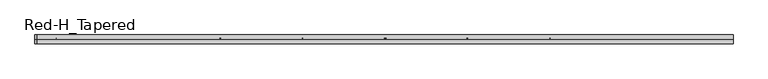
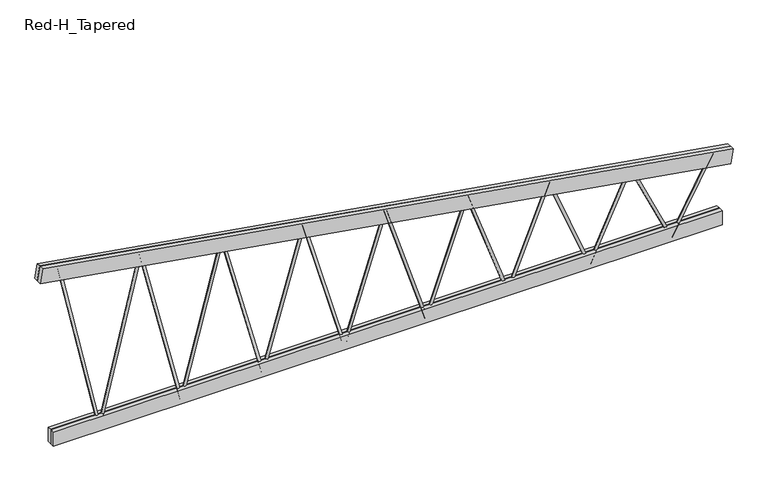
"""IFC4 building model written with IfcOpenShell, lengths in millimetres: beam geometry, Construction_Frames_RedBuilt_Openweb_Red-H_Tapered : Red-H_Tapered."""

from ifc_helpers import new_model, si_unit, point, frame, origin, origin_2d, place, context, project, spatial, polyline, circle_curve, trimmed, segment, composite_curve, outline, extrude, source, transform, mapped, element, save


def red_h_tapered_2805eec2(model_context):
    return source(origin(), model_context, "Body", "SweptSolid", [
        extrude(outline(composite_curve([segment(trimmed(circle_curve(origin_2d(), 12.7), [point((0.0, -12.7))], [point((0.0, 12.7))], False, "CARTESIAN"), True, "CONTINUOUS"), segment(trimmed(circle_curve(origin_2d(), 12.7), [point((0.0, 12.7))], [point((0.0, -12.7))], False, "CARTESIAN"), True, "CONTINUOUS")], self_intersect=False)), frame((-378.61875, 0.0, -417.8101562), z_axis=(-0.277995532529411, 0.0, 0.9605823670532836), x_axis=(0.0, 1.0, 0.0)), (0.0, 0.0, 1.0), 1361.9598364),
        extrude(outline(composite_curve([segment(trimmed(circle_curve(origin_2d(), 12.7), [point((0.0, 12.7))], [point((0.0, -12.7))], False, "CARTESIAN"), True, "CONTINUOUS"), segment(trimmed(circle_curve(origin_2d(), 12.7), [point((0.0, -12.7))], [point((0.0, 12.7))], False, "CARTESIAN"), True, "CONTINUOUS")], self_intersect=False)), frame((-1135.85625, 0.0, -417.8101562), z_axis=(0.27799553252941006, 0.0, 0.9605823670532838), x_axis=(0.0, 1.0, 0.0)), (0.0, 0.0, 1.0), 1361.9598364),
        extrude(outline(composite_curve([segment(trimmed(circle_curve(origin_2d(), 12.7), [point((0.0, -12.7))], [point((0.0, 12.7000001))], False, "CARTESIAN"), True, "CONTINUOUS"), segment(trimmed(circle_curve(origin_2d(), 12.7), [point((0.0, 12.7000001))], [point((0.0, -12.7))], False, "CARTESIAN"), True, "CONTINUOUS")], self_intersect=False)), frame((-1135.85625, 0.0, -417.8101562), z_axis=(-0.2554865755688276, 0.0, 0.966812603198838), x_axis=(0.0, 1.0, 0.0)), (0.0, 0.0, 1.0), 1481.9516413),
        extrude(outline(composite_curve([segment(trimmed(circle_curve(origin_2d(), 12.7), [point((0.0, 12.7))], [point((0.0, -12.7000001))], False, "CARTESIAN"), True, "CONTINUOUS"), segment(trimmed(circle_curve(origin_2d(), 12.7), [point((0.0, -12.7000001))], [point((0.0, 12.7))], False, "CARTESIAN"), True, "CONTINUOUS")], self_intersect=False)), frame((-1893.09375, 0.0, -417.8101562), z_axis=(0.25548657556883586, 0.0, 0.9668126031988359), x_axis=(0.0, 1.0, 0.0)), (0.0, 0.0, 1.0), 1481.9516413),
        extrude(outline(composite_curve([segment(trimmed(circle_curve(origin_2d(), 12.7), [point((0.0, -12.7))], [point((0.0, 12.7))], False, "CARTESIAN"), True, "CONTINUOUS"), segment(trimmed(circle_curve(origin_2d(), 12.7), [point((0.0, 12.7))], [point((0.0, -12.7))], False, "CARTESIAN"), True, "CONTINUOUS")], self_intersect=False)), frame((-1893.09375, 0.0, -417.8101562), z_axis=(-0.23624830304325084, 0.0, 0.9716927185634275), x_axis=(0.0, 1.0, 0.0)), (0.0, 0.0, 1.0), 1602.6305591),
        extrude(outline(composite_curve([segment(trimmed(circle_curve(origin_2d(), 12.7), [point((0.0, 12.7))], [point((0.0, -12.7))], False, "CARTESIAN"), True, "CONTINUOUS"), segment(trimmed(circle_curve(origin_2d(), 12.7), [point((0.0, -12.7))], [point((0.0, 12.7))], False, "CARTESIAN"), True, "CONTINUOUS")], self_intersect=False)), frame((-2650.33125, 0.0, -417.8101562), z_axis=(0.23624830304324398, 0.0, 0.9716927185634292), x_axis=(0.0, 1.0, 0.0)), (0.0, 0.0, 1.0), 1602.6305591),
        extrude(outline(composite_curve([segment(trimmed(circle_curve(origin_2d(), 12.7), [point((0.0, -12.7))], [point((0.0, 12.7))], False, "CARTESIAN"), True, "CONTINUOUS"), segment(trimmed(circle_curve(origin_2d(), 12.7), [point((0.0, 12.7))], [point((0.0, -12.7))], False, "CARTESIAN"), True, "CONTINUOUS")], self_intersect=False)), frame((-2650.33125, 0.0, -417.8101562), z_axis=(-0.21963526223165897, 0.0, 0.9755820578426145), x_axis=(0.0, 1.0, 0.0)), (0.0, 0.0, 1.0), 1723.8522911),
        extrude(outline(composite_curve([segment(trimmed(circle_curve(origin_2d(), 12.7), [point((0.0, -12.7))], [point((0.0, 12.7))], False, "CARTESIAN"), True, "CONTINUOUS"), segment(trimmed(circle_curve(origin_2d(), 12.7), [point((0.0, 12.7))], [point((0.0, -12.7))], False, "CARTESIAN"), True, "CONTINUOUS")], self_intersect=False)), frame((2650.33125, 0.0, -417.8101562), z_axis=(0.48331839774277513, 0.0, 0.8754446449681195), x_axis=(0.0, 1.0, 0.0)), (0.0, 0.0, 1.0), 783.3733451),
        extrude(outline(composite_curve([segment(trimmed(circle_curve(origin_2d(), 12.7), [point((0.0, 12.7))], [point((0.0, -12.7))], False, "CARTESIAN"), True, "CONTINUOUS"), segment(trimmed(circle_curve(origin_2d(), 12.7), [point((0.0, -12.7))], [point((0.0, 12.7))], False, "CARTESIAN"), True, "CONTINUOUS")], self_intersect=False)), frame((2650.33125, 0.0, -417.8101562), z_axis=(-0.4233271479189003, 0.0, 0.9059768903426011), x_axis=(0.0, 1.0, 0.0)), (0.0, 0.0, 1.0), 894.3880681),
        extrude(outline(composite_curve([segment(trimmed(circle_curve(origin_2d(), 12.7), [point((0.0, -12.7))], [point((0.0, 12.7))], False, "CARTESIAN"), True, "CONTINUOUS"), segment(trimmed(circle_curve(origin_2d(), 12.7), [point((0.0, 12.7))], [point((0.0, -12.7))], False, "CARTESIAN"), True, "CONTINUOUS")], self_intersect=False)), frame((1893.09375, 0.0, -417.8101562), z_axis=(0.42332714791889964, 0.0, 0.9059768903426014), x_axis=(0.0, 1.0, 0.0)), (0.0, 0.0, 1.0), 894.3880681),
        extrude(outline(composite_curve([segment(trimmed(circle_curve(origin_2d(), 12.7), [point((0.0, 12.7))], [point((0.0, -12.7))], False, "CARTESIAN"), True, "CONTINUOUS"), segment(trimmed(circle_curve(origin_2d(), 12.7), [point((0.0, -12.7))], [point((0.0, 12.7))], False, "CARTESIAN"), True, "CONTINUOUS")], self_intersect=False)), frame((1893.09375, 0.0, -417.8101562), z_axis=(-0.3754069541599523, 0.0, 0.9268600858642838), x_axis=(0.0, 1.0, 0.0)), (0.0, 0.0, 1.0), 1008.5555044),
        extrude(outline(composite_curve([segment(trimmed(circle_curve(origin_2d(), 12.7), [point((0.0, -12.7))], [point((0.0, 12.7))], False, "CARTESIAN"), True, "CONTINUOUS"), segment(trimmed(circle_curve(origin_2d(), 12.7), [point((0.0, 12.7))], [point((0.0, -12.7))], False, "CARTESIAN"), True, "CONTINUOUS")], self_intersect=False)), frame((1135.85625, 0.0, -417.8101562), z_axis=(0.37540695415995146, 0.0, 0.9268600858642841), x_axis=(0.0, 1.0, 0.0)), (0.0, 0.0, 1.0), 1008.5555044),
        extrude(outline(composite_curve([segment(trimmed(circle_curve(origin_2d(), 12.7), [point((0.0, 12.7))], [point((0.0, -12.7))], False, "CARTESIAN"), True, "CONTINUOUS"), segment(trimmed(circle_curve(origin_2d(), 12.7), [point((0.0, -12.7))], [point((0.0, 12.7))], False, "CARTESIAN"), True, "CONTINUOUS")], self_intersect=False)), frame((1135.85625, 0.0, -417.8101562), z_axis=(-0.3365750833372033, 0.0, 0.9416566323647674), x_axis=(0.0, 1.0, 0.0)), (0.0, 0.0, 1.0), 1124.9161591),
        extrude(outline(composite_curve([segment(trimmed(circle_curve(origin_2d(), 12.7), [point((0.0, -12.7))], [point((0.0, 12.7))], False, "CARTESIAN"), True, "CONTINUOUS"), segment(trimmed(circle_curve(origin_2d(), 12.7), [point((0.0, 12.7))], [point((0.0, -12.7))], False, "CARTESIAN"), True, "CONTINUOUS")], self_intersect=False)), frame((378.61875, 0.0, -417.8101562), z_axis=(0.33657508333720376, 0.0, 0.9416566323647673), x_axis=(0.0, 1.0, 0.0)), (0.0, 0.0, 1.0), 1124.9161591),
        extrude(outline(composite_curve([segment(trimmed(circle_curve(origin_2d(), 12.7), [point((0.0, 12.7))], [point((0.0, -12.6999999))], False, "CARTESIAN"), True, "CONTINUOUS"), segment(trimmed(circle_curve(origin_2d(), 12.7), [point((0.0, -12.6999999))], [point((0.0, 12.7))], False, "CARTESIAN"), True, "CONTINUOUS")], self_intersect=False)), frame((378.61875, 0.0, -417.8101562), z_axis=(-0.3046365038173337, 0.0, 0.952468687433845), x_axis=(0.0, 1.0, 0.0)), (0.0, 0.0, 1.0), 1242.8541729),
        extrude(outline(composite_curve([segment(trimmed(circle_curve(origin_2d(), 12.7), [point((0.0, 12.6999999))], [point((0.0, -12.7))], False, "CARTESIAN"), True, "CONTINUOUS"), segment(trimmed(circle_curve(origin_2d(), 12.7), [point((0.0, -12.7))], [point((0.0, 12.6999999))], False, "CARTESIAN"), True, "CONTINUOUS")], self_intersect=False)), frame((-378.61875, 0.0, -417.8101562), z_axis=(0.30463650381731205, 0.0, 0.952468687433852), x_axis=(0.0, 1.0, 0.0)), (0.0, 0.0, 1.0), 1242.8541729),
        extrude(outline(polyline([(-3100.3875, 41.275), (3100.3875, 41.275), (3100.3875, 3.175), (-3100.3875, 3.175), (-3100.3875, 41.275)])), frame((0.0, 0.0, -436.8601562), z_axis=(0.0, 0.0, 1.0), x_axis=(1.0, 0.0, 0.0)), (0.0, 0.0, 1.0), 139.7),
        extrude(outline(polyline([(-3100.3875, -3.175), (3100.3875, -3.175), (3100.3875, -41.275), (-3100.3875, -41.275), (-3100.3875, -3.175)])), frame((0.0, 0.0, -436.8601562), z_axis=(0.0, 0.0, 1.0), x_axis=(1.0, 0.0, 0.0)), (0.0, 0.0, 1.0), 139.7),
        extrude(outline(polyline([(0.0, 38.1), (6492.222889, 38.1), (6492.222889, 0.0), (0.0, 0.0), (0.0, 38.1)])), frame((-3224.9429596, 3.175, 1203.3387666), z_axis=(0.16431968190823418, 0.0, 0.9864071381217681), x_axis=(0.9864071381217681, 0.0, -0.16431968190823418)), (0.0, 0.0, 1.0), 139.7),
        extrude(outline(polyline([(0.0, 38.1), (6492.222889, 38.1), (6492.222889, 0.0), (0.0, 0.0), (0.0, 38.1)])), frame((-3224.9429596, -41.275, 1203.3387666), z_axis=(0.16431968190823418, 0.0, 0.9864071381217681), x_axis=(0.9864071381217681, 0.0, -0.16431968190823418)), (0.0, 0.0, 1.0), 139.7),
    ])


if __name__ == "__main__":
    model = new_model("IFC4")
    model_context = context("Model", 3, world=origin())
    ifc_project = project(units=[si_unit("LENGTHUNIT", "METRE", prefix="MILLI")], contexts=[model_context])
    site = spatial("IfcSite", under=ifc_project)
    building = spatial("IfcBuilding", under=site)
    placement = place(None, origin())
    red_h_tapered_shape = red_h_tapered_2805eec2(model_context)
    element("IfcBeam", 1, ObjectType="Construction_Frames_RedBuilt_Openweb_Red-H_Tapered : Red-H_Tapered", at=placement, inside=building, context=model_context, shape_type="MappedRepresentation", body=[
        mapped(red_h_tapered_shape, transform((0.0, 0.0, 0.0), x_axis=(1.0, 0.0, 0.0), y_axis=(0.0, 1.0, 0.0), z_axis=(0.0, 0.0, 1.0))),
    ])
    save(model, "model.ifc")

# Revit data of these elements
# Type "Construction_Frames_RedBuilt_Openweb_Red-H_Tapered : Red-H_Tapered"
#   Youtube clip = ""
#   Weight Net (Kg) = "0"
#   Webs = "Up to 2\" diameter tubular steel"
#   Uniformat II Description = ""
#   Uniformat II Code = ""
#   Uniclass 2015 Name = "Softwood trusses"
#   Uniclass 2015 Code = "Pr_20_85_90_81"
#   Uniclass 2.0 Description = "Structural Framing Systems"
#   Uniclass 2.0 Code = "SS-15-10-75"
#   Uniclass 1.4 Description = "Trusses"
#   Uniclass 1.4 Code = "L3523"
#   UNSPSC Code = "30103606"
#   Technical description = "http://www.redbuilt.com/reference/literature-and-other-resources"
#   Region South America = "None"
#   Region Oceania = "None"
#   Region North America = "US"
#   Region Middle East = "None"
#   Region Europe = "None"
#   Region Asia = "None"
#   Region Antarctica = "None"
#   Region Africa = "None"
#   QR code = "http://bimobject.com/redbuilt/product/redbuilt-0003"
#   Product url = "http://www.redbuilt.com/products/default.aspx?id=2"
#   Product group = "Wood Trusses"
#   Product family = "Construction"
#   Product data url = "https://bimobject.com/redbuilt/product/redbuilt-0003"
#   Product certification = ""
#   Product SKU = "redbuilt-0003"
#   Product Page URL = "http://www.redbuilt.com/commercial-systems/red-m-red-h-open-web-trusses"
#   Product Guid = "2c5793f2-6ffb-4665-b825-cf90c048e711"
#   Product Documentation Link = "http://www.redbuilt.com/documents/OW_Guide_2017_07_LowRes_wLinks.pdf"
#   OmniClass Description = "Wood Trusses"
#   OmniClass Code = "23-13 35 19 13 17"
#   NBS Reference Description = ""
#   NBS Reference Code = ""
#   Material secondary = "Steel"
#   Material main = "CHARRED WOOD"
#   Masterformat 2014 Description = "Metal-Web Wood Joists"
#   Masterformat 2014 Code = "06 17 36"
#   Manufacturer name = "RedBuilt"
#   Manufacturer country = "United States"
#   Installation instructions = "http://www.redbuilt.com/documents/Installation_Sheets_Open-Web.pdf"
#   IFC Classification = ""
#   EAN code = ""
#   Design country = "United States"
#   Product Information = "http://redbuilt.com/products/default.aspx?id=2"
#   Model = "Red-H-Tapered"
#   Manufacturer URL = "http://redbuilt.com/"
#   Manufacturer = "RedBuilt™"
#   Description = "Open Web Truss"
#   Date of publishing = "8/17/2010"
#   Contact us = "http://redbuilt.com/contact/"
#   Chords = "Double 1½\" x 5½\" MSR lumber"
#   COBIe Type Category = ""
#   Brand url = "http://www.redbuilt.com"
#   BIMobject main category code = "construction"
#   BIMobject main category = "Construction"
#   BIMobject category code = "construction-frames-trusses"
#   BIMobject category = "Frames & Trusses"
#   Web Radius = 0' - 0 1/2"
#   Web Layout Offset Start [instance default] = 0' - 5"
#   Web Layout Offset End [instance default] = 0' - 5"
#   Web Diameter = 0' - 1"
#   TotalLength [instance default] = 20' - 0"
#   Span Minimum = 4' - 0"
#   Span Maximum = 70' - 0"
#   Span Limit [instance default] = 20' - 0"
#   Nominal width = 0' - 0"
#   Nominal height = 0' - 0"
#   Inner Depth Top [instance default] = 0' - 2.76372"
#   Depth Start [instance default] = 6' - 0"
#   Top Chord Length [instance default] = 20' - 1.19701"
#   TC Extension Start Aux [instance default] = 0' - 0"
#   TC Extension End Aux [instance default] = 0' - 0"
#   T-B Chord Length Difference L [instance default] = 0' - 4"
#   T-B Chord Length Difference [instance default] = 0' - 4"
#   Height 2 [instance default] = 6' - 0"
#   Depth Minimum at Wall = 2' - 0"
#   Depth Maximum at Wall = 6' - 0"
#   Depth Lower End [instance default] = 2' - 0"
#   Depth Higher End [instance default] = 6' - 0"
#   Depth End [instance default] = 2' - 0"
#   Depth 2 [instance default] = 2' - 0"
#   Chord Width = 0' - 3 1/4"
#   Chord Thickness = 0' - 1 1/2"
#   Chord Depth = 0' - 5 1/2"
#   Offset Start [instance default] = 0' - 0"
#   TC Extension Start [instance default] = 0' - 0"
#   End Panel = 0' - 5"
#   Offset End [instance default] = 0' - 0"
#   TC Extension End [instance default] = 0' - 0"
#   Length [instance default] = 20' - 0"
#   Angle [instance default] = 5.71059°
#   Span Limit Warning [instance default] = no
#   Edition number = 1
#   Top Bearing Start [instance default] = yes
#   Top Bearing End [instance default] = yes
#   Bottom Bearing Start [instance default] = no
#   Bottom Bearing End [instance default] = no
#   8 Panels [instance default] = yes
#   16 Panels [instance default] = no
#   12 Panels [instance default] = no
#   Web Material = RedBuilt-Steel, Galvanized
#   Clip Material = RedBuilt-Steel, Galvanized
#   Chords Material = WOOD-OAKFIRE
#   URL = ""
#   Assembly Code = ""
# Element 1 (IfcBeam, "Construction_Frames_RedBuilt_Openweb_Red-H_Tapered : Red-H_Tapered")
#   TotalLength = 20' - 8 1/2"
#   Span Limit = 20' - 8 1/2"
#   Inner Depth Top = 0' - 2.789"
#   Depth Start = 5' - 0"
#   Top Chord Length = 21' - 0.0243"
#   Height 2 = 5' - 0"
#   Depth Lower End = 2' - 4"
#   Depth Higher End = 5' - 0"
#   Depth End = 2' - 4"
#   Depth 2 = 3' - 6"
#   Angle = 9.59313°
#   Materials on its faces: "RedBuilt-Steel, Galvanized", "WOOD-OAKFIRE"
# Materials
#   "RedBuilt-Steel, Galvanized": class "Metal", colour RGB 164 172 176, transparency 0, Manufacturer = "RedBuilt. LLC", Comments = "Openweb Metal Web", URL = "http://www.redbuilt.com/", Description = "Galvanized steel", Cost = 0
#   "WOOD-OAKFIRE": class "Wood", colour RGB 198 202 183, transparency 0, Description = "Generic wood", Cost = 0
